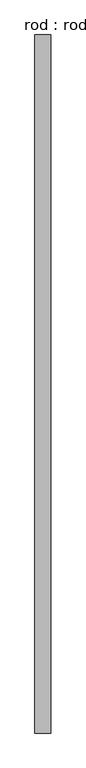
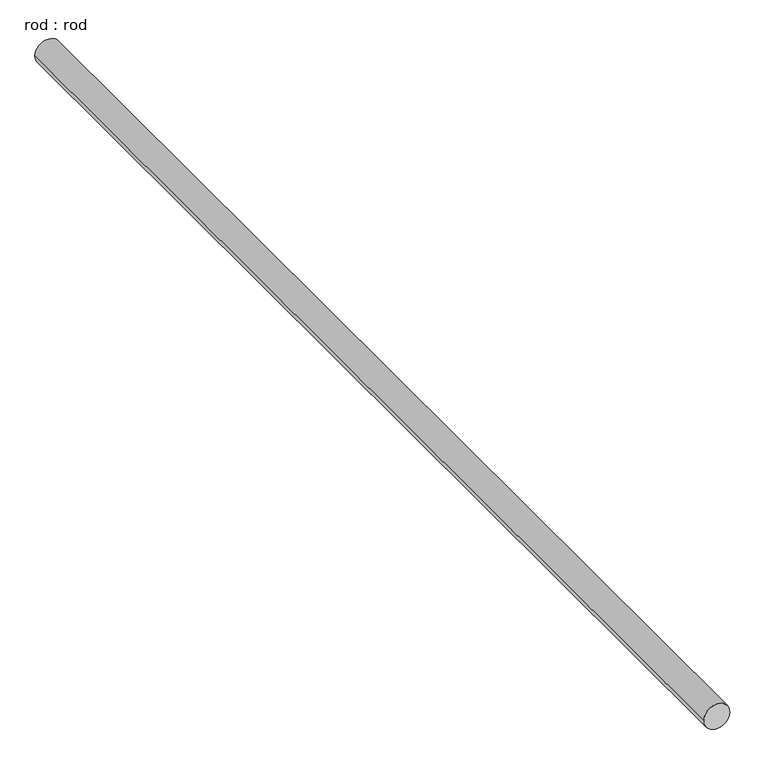
"""IFC4 building model written with IfcOpenShell, lengths in millimetres: proxy geometry, rod : rod."""

from ifc_helpers import new_model, si_unit, point, frame, frame_2d, origin, place, context, project, spatial, circle_curve, trimmed, segment, composite_curve, outline, extrude, source, transform, mapped, element, save


def rod_rod_65bb73e3(model_context):
    return source(origin(), model_context, "Body", "SweptSolid", [
        extrude(outline(composite_curve([segment(trimmed(circle_curve(frame_2d((0.0108462, 0.0)), 200.0), [point((0.0108462, 200.0))], [point((0.0108462, -200.0))], False, "CARTESIAN"), True, "CONTINUOUS"), segment(trimmed(circle_curve(frame_2d((0.0108462, 0.0)), 200.0), [point((0.0108462, -200.0))], [point((0.0108462, 200.0))], False, "CARTESIAN"), True, "CONTINUOUS")], self_intersect=False)), frame((0.0, -4758.6906471, 0.0), z_axis=(0.0, 1.0, 0.0), x_axis=(0.0, 0.0, 1.0)), (0.0, 0.0, 1.0), 17702.8385248),
    ])


if __name__ == "__main__":
    model = new_model("IFC4")
    model_context = context("Model", 3, world=origin())
    ifc_project = project(units=[si_unit("LENGTHUNIT", "METRE", prefix="MILLI")], contexts=[model_context])
    site = spatial("IfcSite", under=ifc_project)
    building = spatial("IfcBuilding", under=site)
    placement = place(None, origin())
    rod_rod_shape = rod_rod_65bb73e3(model_context)
    element("IfcBuildingElementProxy", 1, Name="rod : rod", ObjectType="rod : rod", at=placement, inside=building, context=model_context, shape_type="MappedRepresentation", body=[
        mapped(rod_rod_shape, transform((0.0, 0.0, 0.0), x_axis=(1.0, 0.0, 0.0), y_axis=(0.0, 1.0, 0.0), z_axis=(0.0, 0.0, 1.0))),
    ])
    save(model, "model.ifc")

# Revit data of these elements
# Type "rod : rod"
#   Default Elevation = 0
